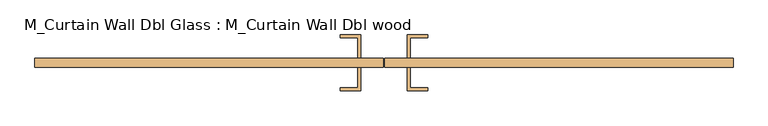
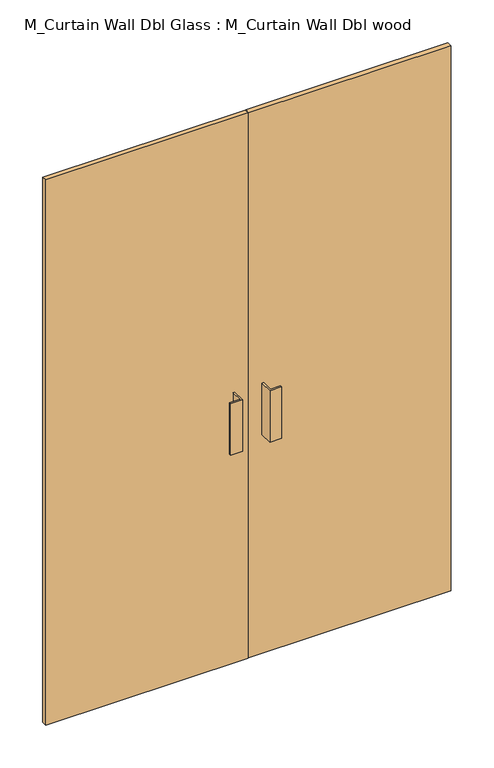
"""IFC4 building model written with IfcOpenShell, lengths in millimetres: door geometry, M_Curtain Wall Dbl Glass : M_Curtain Wall Dbl wood."""

from ifc_helpers import new_model, si_unit, frame, origin, origin_with_axes, place, context, project, spatial, polyline, outline, extrude, source, transform, mapped, element, save


def m_curtain_wall_dbl_glass_m_curtain_wall_dbl_wood_a5b828f6(model_context):
    return source(origin(), model_context, "Body", "SweptSolid", [
        extrude(outline(polyline([(-1.5875, 19.05), (-1.5875, 0.0), (-756.3789943, 0.0), (-756.3789943, 19.05), (-1.5875, 19.05)])), origin_with_axes(), (0.0, 0.0, 1.0), 2150.0),
        extrude(outline(polyline([(756.3789943, 19.05), (756.3789943, 0.0), (1.5875, 0.0), (1.5875, 19.05), (756.3789943, 19.05)])), origin_with_axes(), (0.0, 0.0, 1.0), 2150.0),
        extrude(outline(polyline([(-50.8, -50.8), (-95.25, -50.8), (-95.25, -44.45), (-57.15, -44.45), (-57.15, 0.0), (-50.8, 0.0), (-50.8, -50.8)])), frame((0.0, 0.0, 863.6), z_axis=(0.0, 0.0, 1.0), x_axis=(1.0, 0.0, 0.0)), (0.0, 0.0, 1.0), 203.2),
        extrude(outline(polyline([(50.8, -50.8), (50.8, 0.0), (57.15, 0.0), (57.15, -44.45), (95.25, -44.45), (95.25, -50.8), (50.8, -50.8)])), frame((0.0, 0.0, 863.6), z_axis=(0.0, 0.0, 1.0), x_axis=(1.0, 0.0, 0.0)), (0.0, 0.0, 1.0), 203.2),
        extrude(outline(polyline([(-50.8, 69.85), (-50.8, 19.05), (-57.15, 19.05), (-57.15, 63.5), (-95.25, 63.5), (-95.25, 69.85), (-50.8, 69.85)])), frame((0.0, 0.0, 863.6), z_axis=(0.0, 0.0, 1.0), x_axis=(1.0, 0.0, 0.0)), (0.0, 0.0, 1.0), 203.2),
        extrude(outline(polyline([(50.8, 69.85), (95.25, 69.85), (95.25, 63.5), (57.15, 63.5), (57.15, 19.05), (50.8, 19.05), (50.8, 69.85)])), frame((0.0, 0.0, 863.6), z_axis=(0.0, 0.0, 1.0), x_axis=(1.0, 0.0, 0.0)), (0.0, 0.0, 1.0), 203.2),
    ])


if __name__ == "__main__":
    model = new_model("IFC4")
    model_context = context("Model", 3, world=origin())
    ifc_project = project(units=[si_unit("LENGTHUNIT", "METRE", prefix="MILLI")], contexts=[model_context])
    site = spatial("IfcSite", under=ifc_project)
    building = spatial("IfcBuilding", under=site)
    placement = place(None, origin())
    m_curtain_wall_dbl_glass_m_curtain_wall_dbl_wood_shape = m_curtain_wall_dbl_glass_m_curtain_wall_dbl_wood_a5b828f6(model_context)
    element("IfcDoor", 1, ObjectType="M_Curtain Wall Dbl Glass : M_Curtain Wall Dbl wood", at=placement, inside=building, context=model_context, shape_type="MappedRepresentation", body=[
        mapped(m_curtain_wall_dbl_glass_m_curtain_wall_dbl_wood_shape, transform((0.0, 0.0, 0.0), x_axis=(1.0, 0.0, 0.0), y_axis=(0.0, 1.0, 0.0), z_axis=(0.0, 0.0, 1.0))),
    ])
    save(model, "model.ifc")

# Revit data of these elements
# Type "M_Curtain Wall Dbl Glass : M_Curtain Wall Dbl wood"
#   Model = "12345679"
#   Manufacturer = "Dublin Doors"
#   Description = "Double Wood Door"
#   Type Mark = "46"
#   Fire Rating = "60M"
#   COBie.Type.CreatedBy = "design@eagle.com"
#   COBie.Type.CreatedOn = "2016-09-13T05:47:35"
#   COBie.Type.Name = "Doors_M_Curtain Wall Dbl Glass_M_Curtain Wall Dbl wood"
#   COBie.Type.Category = "23-30 10 00 : Doors"
#   COBie.Type.Description = "Double Wood Door"
#   COBie.Type.Manufacturer = "Dublin Doors"
#   COBie.Type.ModelNumber = "12345679"
#   Construction Type Id = "opn-d36"
#   Analytic Construction = "Wood panel"
#   COBie.Type.ReplacementCost = 0
#   Offset = 0 mm
#   Heat Transfer Coefficient (U) = 3.8042 W/(m²·K)
#   COBie.Type = yes
#   Function = 1
#   Glazing Material = Door - Panel
#   Visual Light Transmittance = 0
#   Solar Heat Gain Coefficient = 0
# Element 1 (IfcDoor, "M_Curtain Wall Dbl Glass : M_Curtain Wall Dbl wood")
#   Materials on its faces: "Aluminum", "Door - Panel"
# Materials
#   "Door - Panel": class "Wood", colour RGB 210 159 95, transparency 0
#   "Aluminum": class "Metal", colour RGB 247 247 247, transparency 0, Description = "Aluminum 6061", Cost = 0
